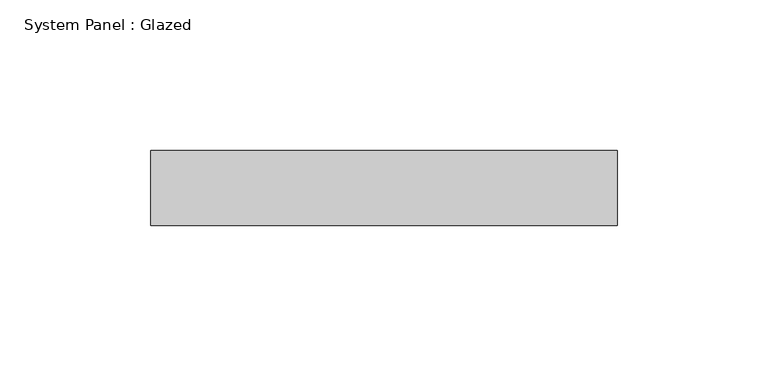
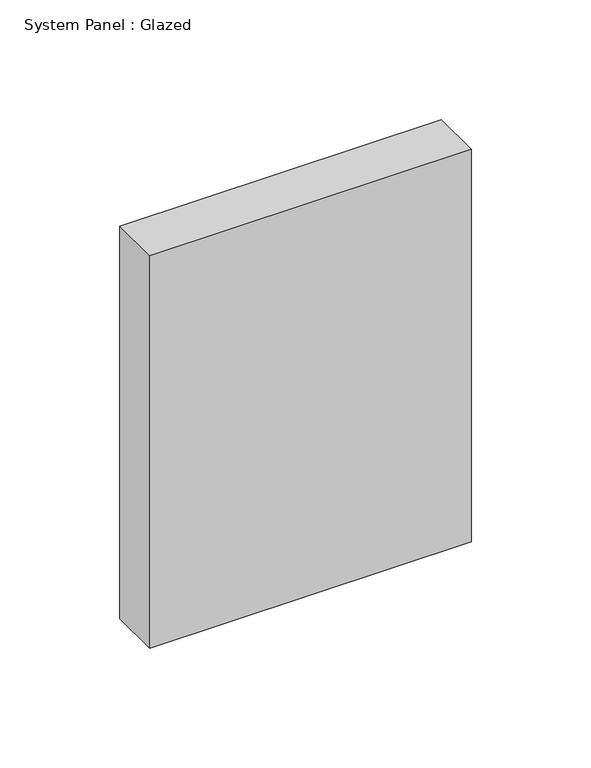
"""IFC4 building model written with IfcOpenShell, lengths in millimetres: plate geometry, System Panel : Glazed."""

from ifc_helpers import new_model, si_unit, origin, origin_with_axes, place, context, project, spatial, polyline, outline, extrude, source, transform, mapped, element, save


def system_panel_glazed_83ffeb2f(model_context):
    return source(origin(), model_context, "Body", "SweptSolid", [
        extrude(outline(polyline([(77.5306965, 24.5), (-77.5306965, 24.5), (-77.5306965, 49.5), (77.5306965, 49.5), (77.5306965, 24.5)])), origin_with_axes(), (0.0, 0.0, 1.0), 200.0),
    ])


if __name__ == "__main__":
    model = new_model("IFC4")
    model_context = context("Model", 3, world=origin())
    ifc_project = project(units=[si_unit("LENGTHUNIT", "METRE", prefix="MILLI")], contexts=[model_context])
    site = spatial("IfcSite", under=ifc_project)
    building = spatial("IfcBuilding", under=site)
    placement = place(None, origin())
    system_panel_glazed_shape = system_panel_glazed_83ffeb2f(model_context)
    element("IfcPlate", 1, ObjectType="System Panel : Glazed", at=placement, inside=building, context=model_context, shape_type="MappedRepresentation", body=[
        mapped(system_panel_glazed_shape, transform((0.0, 0.0, 0.0), x_axis=(1.0, 0.0, 0.0), y_axis=(0.0, 1.0, 0.0), z_axis=(0.0, 0.0, 1.0))),
    ])
    save(model, "model.ifc")

# Revit data of these elements
# Element 1 (IfcPlate, "System Panel : Glazed")
#   Materials on its faces: "Glass"
# Materials
#   "Glass": class "Glass", colour RGB 218 227 224, transparency 0.85, Description = "Soda Lime Glass", Cost = 0
